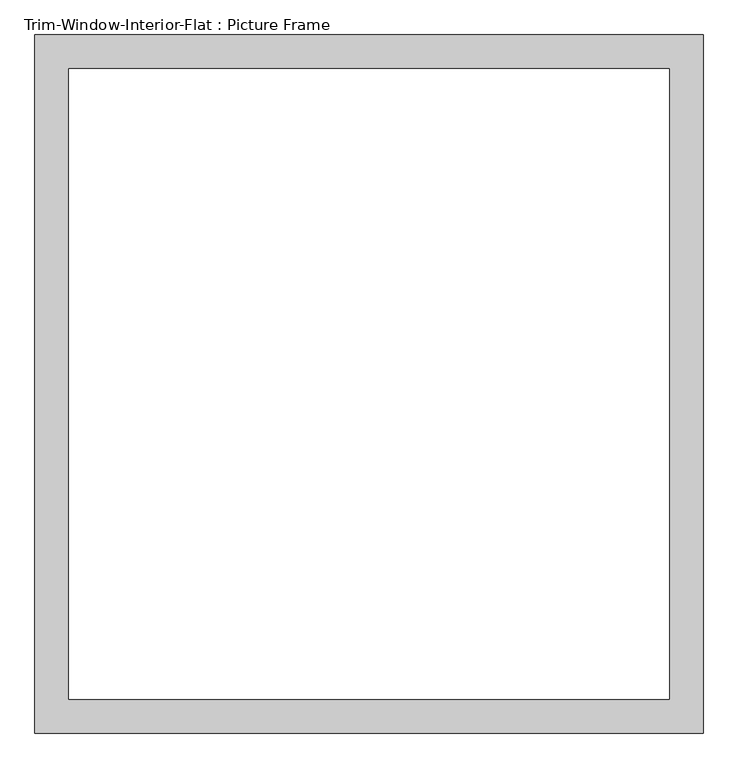
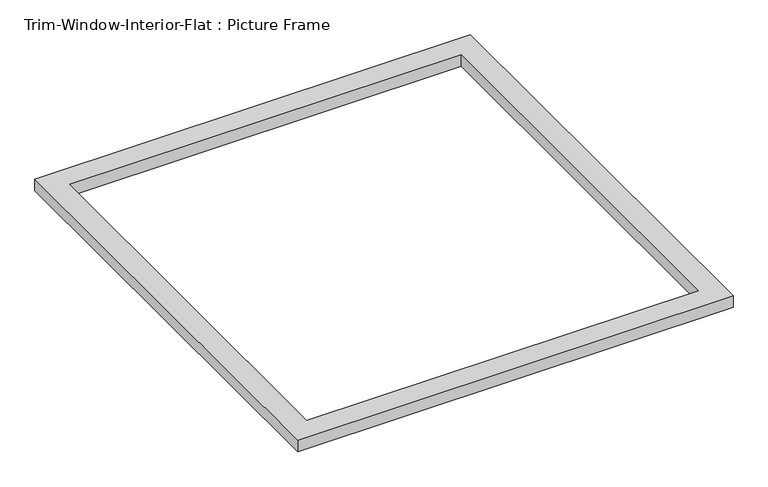
"""IFC4 building model written with IfcOpenShell, lengths in millimetres: proxy geometry, Trim-Window-Interior-Flat : Picture Frame."""

from ifc_helpers import new_model, si_unit, origin, origin_with_axes, place, context, project, spatial, polyline, outline, extrude, source, transform, mapped, element, save


def trim_window_interior_flat_picture_frame_be940afe(model_context):
    return source(origin(), model_context, "Body", "SweptSolid", [
        extrude(outline(polyline([(565.15, 44.45), (565.15, -1136.65), (-565.15, -1136.65), (-565.15, 44.45), (565.15, 44.45)]), holes=[polyline([(508.0, -12.7), (-508.0, -12.7), (-508.0, -1079.5), (508.0, -1079.5), (508.0, -12.7)])]), origin_with_axes(), (0.0, 0.0, 1.0), 31.75),
    ])


if __name__ == "__main__":
    model = new_model("IFC4")
    model_context = context("Model", 3, world=origin())
    ifc_project = project(units=[si_unit("LENGTHUNIT", "METRE", prefix="MILLI")], contexts=[model_context])
    site = spatial("IfcSite", under=ifc_project)
    building = spatial("IfcBuilding", under=site)
    placement = place(None, origin())
    trim_window_interior_flat_picture_frame_shape = trim_window_interior_flat_picture_frame_be940afe(model_context)
    element("IfcBuildingElementProxy", 1, Name="Trim-Window-Interior-Flat : Picture Frame", ObjectType="Trim-Window-Interior-Flat : Picture Frame", at=placement, inside=building, context=model_context, shape_type="MappedRepresentation", body=[
        mapped(trim_window_interior_flat_picture_frame_shape, transform((0.0, 0.0, 0.0), x_axis=(1.0, 0.0, 0.0), y_axis=(0.0, 1.0, 0.0), z_axis=(0.0, 0.0, 1.0))),
    ])
    save(model, "model.ifc")

# Revit data of these elements
# Type "Trim-Window-Interior-Flat : Picture Frame"
#   Trim Thickness_Picture Frame = 0' - 1 1/4"
#   Trim Width = 0' - 2 1/4"
#   Trim Thickness_with Sill = 0' - 0 3/4"
#   Sill Thickness = 0' - 1 1/4"
#   Opening Width [instance default] = 2' - 0"
#   Opening Height [instance default] = 3' - 0"
#   Default Elevation = 4' - 0"
#   Sill = no
#   Picture Frame = yes
#   Trim Material [instance default] = none
# Element 1 (IfcBuildingElementProxy, "Trim-Window-Interior-Flat : Picture Frame")
#   Opening Width = 3' - 5"
#   Opening Height = 3' - 7"
#   Trim Material = 1X WOOD COMPOSITE TRIM
#   Materials on its faces: "1X WOOD COMPOSITE TRIM"
# Materials
#   "1X WOOD COMPOSITE TRIM": class "Generic", colour RGB 88 61 61, transparency 0, Cost = 0
